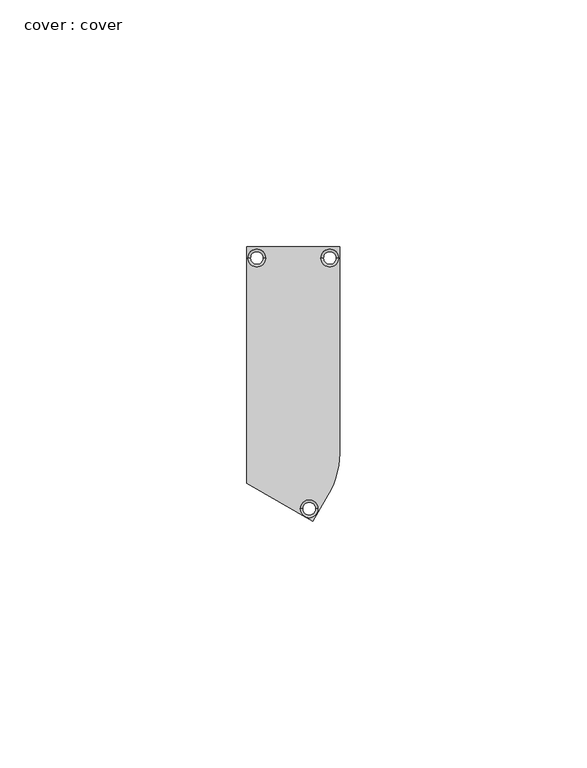
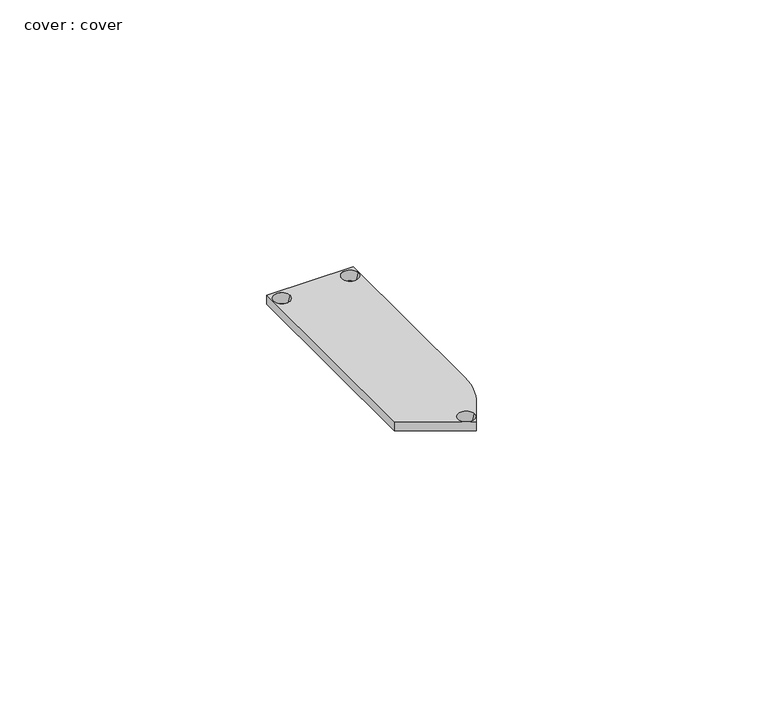
"""IFC4 building model written with IfcOpenShell, lengths in millimetres: proxy geometry, cover : cover."""

import ifcopenshell
import ifcopenshell.guid

model = None  # the IFC model being written
_history = None  # IfcOwnerHistory: only IFC2X3 demands one
_inside = {}  # id of a spatial element -> (the spatial element, [elements in it])
_under = {}  # id of a project, library or spatial element -> (it, [spatial elements below it])
_declared = {}  # id of a project -> (the project, [libraries it declares])
_typed = {}  # id of a type object -> (the type object, [elements of that type])
_made_of = {}  # id of a material, layer set ... -> (it, [elements and type objects made of it])


def new_model(schema):
    """Start an empty IFC model of exactly this schema.

    Asked for "IFC4X3", IfcOpenShell would pick the latest addendum, in which some entities
    have other attributes; the version numbers below select the first issue.
    IFC2X3 requires an IfcOwnerHistory on every rooted entity: one is made here for all.
    """
    global model, _history
    if schema == "IFC4X3":
        model = ifcopenshell.file(schema_version=(4, 3, 0, 0))
    else:
        model = ifcopenshell.file(schema=schema)
    _inside.clear()
    _under.clear()
    _declared.clear()
    _typed.clear()
    _made_of.clear()
    _history = None
    if model.schema == "IFC2X3":
        org = make("IfcOrganization", Name="unknown")
        user = make(
            "IfcPersonAndOrganization",
            ThePerson=make("IfcPerson", FamilyName="unknown"),
            TheOrganization=org,
        )
        app = make(
            "IfcApplication",
            ApplicationDeveloper=org,
            Version="unknown",
            ApplicationFullName="unknown",
            ApplicationIdentifier="unknown",
        )
        _history = make(
            "IfcOwnerHistory",
            OwningUser=user,
            OwningApplication=app,
            ChangeAction="ADDED",
            CreationDate=0,
        )
    return model


def make(cls, **values):
    """One entity of the class cls with the attributes given. An attribute that is None is left unset."""
    return model.create_entity(
        cls, **{name: value for name, value in values.items() if value is not None}
    )


def rooted(cls, **values):
    """An entity with a GlobalId (a new one), such as an element, a storey or a relation."""
    return make(cls, GlobalId=ifcopenshell.guid.new(), OwnerHistory=_history, **values)


def si_unit(unit_type, name, prefix=None):
    """IfcSIUnit, for example si_unit("LENGTHUNIT", "METRE", prefix="MILLI")."""
    return make("IfcSIUnit", UnitType=unit_type, Prefix=prefix, Name=name)


def assignment(units):
    """IfcUnitAssignment: the units of a project."""
    return None if units is None else make("IfcUnitAssignment", Units=units)


def point(xyz):
    """IfcCartesianPoint."""
    return None if xyz is None else make("IfcCartesianPoint", Coordinates=xyz)


def direction(xyz):
    """IfcDirection."""
    return None if xyz is None else make("IfcDirection", DirectionRatios=xyz)


def frame(location, z_axis=None, x_axis=None):
    """IfcAxis2Placement3D, a coordinate frame: its origin and axes. An axis left out is left unset."""
    return make(
        "IfcAxis2Placement3D",
        Location=point(location),
        Axis=direction(z_axis),
        RefDirection=direction(x_axis),
    )


def origin():
    """The frame at (0, 0, 0) with its axes left unset."""
    return frame((0.0, 0.0, 0.0))


def place(relative_to, where):
    """IfcLocalPlacement: puts the frame where relative to a parent placement (None: the world)."""
    return make(
        "IfcLocalPlacement", PlacementRelTo=relative_to, RelativePlacement=where
    )


def context(
    kind, dimensions, precision=None, world=None, true_north=None, identifier=None
):
    """IfcGeometricRepresentationContext, for example the 3D "Model" context."""
    return make(
        "IfcGeometricRepresentationContext",
        ContextIdentifier=identifier,
        ContextType=kind,
        CoordinateSpaceDimension=dimensions,
        Precision=precision,
        WorldCoordinateSystem=world,
        TrueNorth=true_north,
    )


def project(units=None, contexts=None):
    """IfcProject with its units and contexts."""
    return rooted(
        "IfcProject",
        Name="project",
        RepresentationContexts=contexts,
        UnitsInContext=assignment(units),
    )


def spatial(cls, under=None, at=None, **own):
    """A site, building, storey or space (cls), placed at a placement, below another one or the project."""
    s = rooted(cls, ObjectPlacement=at, **own)
    if under is not None:
        _under.setdefault(under.id(), (under, []))[1].append(s)
    return s


def polyline(points):
    """IfcPolyline through the points."""
    return make("IfcPolyline", Points=[point(p) for p in points])


def circle_curve(where, radius):
    """IfcCircle in the frame where."""
    return make("IfcCircle", Position=where, Radius=radius)


def shape(context_of_items, identifier, shape_type, items):
    """IfcShapeRepresentation: the items that make up one representation, for example the "Body"."""
    return make(
        "IfcShapeRepresentation",
        ContextOfItems=context_of_items,
        RepresentationIdentifier=identifier,
        RepresentationType=shape_type,
        Items=items,
    )


def source(mapping_origin, context_of_items, identifier, shape_type, items):
    """IfcRepresentationMap: a shape defined once, which mapped items show again and again."""
    return make(
        "IfcRepresentationMap",
        MappingOrigin=mapping_origin,
        MappedRepresentation=shape(context_of_items, identifier, shape_type, items),
    )


def transform(
    local_origin,
    x_axis=None,
    y_axis=None,
    z_axis=None,
    scale=None,
    scale2=None,
    scale3=None,
    uniform=True,
):
    """IfcCartesianTransformationOperator3D, or its non-uniform kind. x_axis, y_axis, z_axis: its Axis1, 2, 3."""
    if uniform:
        return make(
            "IfcCartesianTransformationOperator3D",
            Axis1=direction(x_axis),
            Axis2=direction(y_axis),
            LocalOrigin=point(local_origin),
            Scale=scale,
            Axis3=direction(z_axis),
        )
    return make(
        "IfcCartesianTransformationOperator3DnonUniform",
        Axis1=direction(x_axis),
        Axis2=direction(y_axis),
        LocalOrigin=point(local_origin),
        Scale=scale,
        Axis3=direction(z_axis),
        Scale2=scale2,
        Scale3=scale3,
    )


def mapped(mapping_source, mapping_target):
    """IfcMappedItem: shows the shape of a source again, moved by a transform."""
    return make(
        "IfcMappedItem", MappingSource=mapping_source, MappingTarget=mapping_target
    )


def made_of(thing, what):
    """Note that an element or type object is made of a material, layer set ...; save() writes the relation."""
    if what is not None:
        _made_of.setdefault(what.id(), (what, []))[1].append(thing)
    return thing


def element(
    cls,
    number,
    at=None,
    inside=None,
    cuts=None,
    type_object=None,
    material=None,
    context=None,
    identifier="Body",
    shape_type=None,
    held_by="IfcProductDefinitionShape",
    body=None,
    shapes=None,
    **own,
):
    """One element of the class cls, such as IfcWall. Its Tag is "e" and its number.

    at: its placement. inside: the storey or other place that contains it. cuts: it is an
    opening in that element (IfcRelVoidsElement). A single representation is given by context,
    identifier, shape_type and body (its items); several are given by shapes. held_by: the class
    of the entity that holds the representations. save() writes the other relations.
    """
    e = rooted(cls, Tag="e%d" % number, ObjectPlacement=at, **own)
    if body is not None:
        shapes = [shape(context, identifier, shape_type, body)]
    if shapes is not None:
        e.Representation = make(held_by, Representations=shapes)
    if inside is not None:
        _inside.setdefault(inside.id(), (inside, []))[1].append(e)
    if cuts is not None:
        rooted(
            "IfcRelVoidsElement", RelatingBuildingElement=cuts, RelatedOpeningElement=e
        )
    if type_object is not None:
        _typed.setdefault(type_object.id(), (type_object, []))[1].append(e)
    return made_of(e, material)


def aggregate(whole, parts):
    """IfcRelAggregates: a whole, such as a stair, and the parts it consists of."""
    return rooted("IfcRelAggregates", RelatingObject=whole, RelatedObjects=parts)


def save(model, path):
    """Write the relations noted so far, then the file.

    IfcRelAggregates (storeys below a building ...), IfcRelContainedInSpatialStructure (elements
    in a storey), IfcRelDefinesByType, IfcRelAssociatesMaterial and IfcRelDeclares: one each for
    every whole, place, type object, material and project.
    """
    for whole, parts in _under.values():
        aggregate(whole, parts)
    for where, things in _inside.values():
        rooted(
            "IfcRelContainedInSpatialStructure",
            RelatedElements=things,
            RelatingStructure=where,
        )
    for kind, things in _typed.values():
        rooted("IfcRelDefinesByType", RelatedObjects=things, RelatingType=kind)
    for what, things in _made_of.values():
        rooted("IfcRelAssociatesMaterial", RelatedObjects=things, RelatingMaterial=what)
    for by, libraries in _declared.values():
        rooted("IfcRelDeclares", RelatingContext=by, RelatedDefinitions=libraries)
    model.write(path)


def plane_surface(at):
    """IfcPlane: the flat surface through the origin of the frame at, square to its z axis."""
    return make("IfcPlane", Position=at)


def revolved_surface(curve, axis_point, axis_direction):
    """IfcSurfaceOfRevolution: the curve turned about the line through axis_point along axis_direction."""
    return make(
        "IfcSurfaceOfRevolution",
        SweptCurve=make("IfcArbitraryOpenProfileDef", ProfileType="CURVE", Curve=curve),
        AxisPosition=make("IfcAxis1Placement", Location=point(axis_point), Axis=direction(axis_direction)),
    )


def advanced_brep(points, edges, surfaces, faces):
    """IfcAdvancedBrep: a solid bounded by faces that lie on surfaces and meet in shared edges.

    An edge is (start, end): straight between two places in points (the first is 0);
    or (start, end, curve); or (start, end, curve, False) where it runs against its curve.
    A face is (place in surfaces, loops), or (place, loops, False) where it looks against
    its surface's normal. A loop lists edges by number (the first is 1), with a minus sign
    where the edge is run from its end to its start. The first loop is the outer one.
    """
    corners = [point(p) for p in points]
    vertices = [make("IfcVertexPoint", VertexGeometry=c) for c in corners]
    made = []
    for start, end, *more in edges:
        made.append(
            make(
                "IfcEdgeCurve",
                EdgeStart=vertices[start],
                EdgeEnd=vertices[end],
                EdgeGeometry=more[0] if more else make("IfcPolyline", Points=[corners[start], corners[end]]),
                SameSense=more[1] if len(more) > 1 else True,
            )
        )
    hull = []
    for where, loops, *sense in faces:
        bounds = []
        for j, loop in enumerate(loops):
            ring = [make("IfcOrientedEdge", EdgeElement=made[abs(k) - 1], Orientation=k > 0) for k in loop]
            bounds.append(
                make(
                    "IfcFaceOuterBound" if j == 0 else "IfcFaceBound",
                    Bound=make("IfcEdgeLoop", EdgeList=ring),
                    Orientation=True,
                )
            )
        hull.append(make("IfcAdvancedFace", Bounds=bounds, FaceSurface=surfaces[where], SameSense=sense[0] if sense else True))
    return make("IfcAdvancedBrep", Outer=make("IfcClosedShell", CfsFaces=hull))


def cover_cover_f3c25fb8(model_context):
    return source(origin(), model_context, "Body", "AdvancedBrep", [
        advanced_brep(
        [(4663.3311724, 3578.6670305, 2.0), (4663.3311724, 3530.8564939, 2.0), (4676.6686902, 3523.1530364, 2.0), (4680.3669524, 3529.5586705, 2.0), (4680.8851124, 3530.7118305, 2.0), (4681.3143724, 3531.9030905, 2.0), (4681.6547324, 3533.1222905, 2.0), (4681.9011124, 3534.3618105, 2.0), (4682.0560524, 3535.6191105, 2.0), (4682.1119324, 3536.8840305, 2.0), (4682.1119324, 3578.6670305, 2.0), (4667.1314224, 3576.4165905, 2.0), (4663.5314224, 3576.4165905, 2.0), (4681.9129524, 3576.4165905, 2.0), (4678.3129524, 3576.4165905, 2.0), (4677.7131366, 3525.6369105, 2.0), (4674.1587083, 3525.6369105, 2.0), (4663.3311724, 3578.6670305, 0.0), (4682.1119324, 3578.6670305, 0.0), (4682.1119324, 3536.8840305, 0.0), (4682.0560524, 3535.6191105, 0.0), (4681.9011124, 3534.3618105, 0.0), (4681.6547324, 3533.1222905, 0.0), (4681.3143724, 3531.9030905, 0.0), (4680.8851124, 3530.7118305, 0.0), (4680.3669524, 3529.5586705, 0.0), (4676.6686902, 3523.1530364, 0.0), (4663.3311724, 3530.8564939, 0.0), (4664.0314224, 3576.4165905, 0.0), (4666.6314224, 3576.4165905, 0.0), (4678.8129524, 3576.4165905, 0.0), (4681.4129524, 3576.4165905, 0.0), (4674.6206691, 3525.6369105, 0.0), (4677.2511758, 3525.6369105, 0.0)],
        [
            (0, 1),
            (1, 2),
            (2, 3),
            (3, 4),
            (4, 5),
            (5, 6),
            (6, 7),
            (7, 8),
            (8, 9),
            (9, 10),
            (10, 0),
            (11, 12, circle_curve(frame((4665.3314224, 3576.4165905, 2.0), z_axis=(0.0, 0.0, -1.0), x_axis=(-1.0, 0.0, 0.0)), 1.8)),
            (12, 11, circle_curve(frame((4665.3314224, 3576.4165905, 2.0), z_axis=(0.0, 0.0, -1.0), x_axis=(1.0, 0.0, 0.0)), 1.8)),
            (13, 14, circle_curve(frame((4680.1129524, 3576.4165905, 2.0), z_axis=(0.0, 0.0, -1.0), x_axis=(-1.0, 0.0, 0.0)), 1.8)),
            (14, 13, circle_curve(frame((4680.1129524, 3576.4165905, 2.0), z_axis=(0.0, 0.0, -1.0), x_axis=(1.0, 0.0, 0.0)), 1.8)),
            (15, 16, circle_curve(frame((4675.9359224, 3525.6369105, 2.0), z_axis=(0.0, 0.0, -1.0), x_axis=(-1.0, 0.0, 0.0)), 1.7772142)),
            (16, 15, circle_curve(frame((4675.9359224, 3525.6369105, 2.0), z_axis=(0.0, 0.0, -1.0), x_axis=(1.0, 0.0, 0.0)), 1.7772142)),
            (17, 18),
            (18, 19),
            (19, 20),
            (20, 21),
            (21, 22),
            (22, 23),
            (23, 24),
            (24, 25),
            (25, 26),
            (26, 27),
            (27, 17),
            (28, 29, circle_curve(frame((4665.3314224, 3576.4165905, 0.0), z_axis=(0.0, 0.0, 1.0), x_axis=(-1.0, 0.0, 0.0)), 1.3)),
            (29, 28, circle_curve(frame((4665.3314224, 3576.4165905, 0.0), z_axis=(0.0, 0.0, 1.0), x_axis=(1.0, 0.0, 0.0)), 1.3)),
            (30, 31, circle_curve(frame((4680.1129524, 3576.4165905, 0.0), z_axis=(0.0, 0.0, 1.0), x_axis=(-1.0, 0.0, 0.0)), 1.3)),
            (31, 30, circle_curve(frame((4680.1129524, 3576.4165905, 0.0), z_axis=(0.0, 0.0, 1.0), x_axis=(1.0, 0.0, 0.0)), 1.3)),
            (32, 33, circle_curve(frame((4675.9359224, 3525.6369105, 0.0), z_axis=(0.0, 0.0, 1.0), x_axis=(-1.0, 0.0, 0.0)), 1.3152534)),
            (33, 32, circle_curve(frame((4675.9359224, 3525.6369105, 0.0), z_axis=(0.0, 0.0, 1.0), x_axis=(1.0, 0.0, 0.0)), 1.3152534)),
            (0, 17),
            (27, 1),
            (26, 2),
            (25, 3),
            (9, 19),
            (18, 10),
            (24, 4),
            (23, 5),
            (22, 6),
            (21, 7),
            (20, 8),
            (28, 12),
            (11, 29),
            (30, 14),
            (13, 31),
            (32, 16),
            (15, 33),
        ],
        [
            plane_surface(frame((4663.3311724, 3531.8548305, 2.0), z_axis=(0.0, 0.0, 1.0), x_axis=(0.0, -1.0, 0.0))),
            plane_surface(frame((4663.3311724, 3531.8548305, 0.0), z_axis=(0.0, 0.0, -1.0), x_axis=(0.0, 1.0, 0.0))),
            plane_surface(frame((4663.3311724, 3578.6670305, 2.0), z_axis=(-1.0, 0.0, 0.0), x_axis=(0.0, 0.0, -1.0))),
            plane_surface(frame((4663.3311724, 3530.8564939, 2.0), z_axis=(-0.5001479267947538, -0.8659399813629751, 0.0), x_axis=(0.0, 0.0, -1.0))),
            plane_surface(frame((4676.6686902, 3523.1530364, 2.0), z_axis=(0.8660272939548952, -0.49999672611444335, 0.0), x_axis=(0.0, 0.0, -1.0))),
            plane_surface(frame((4682.1119324, 3536.8840305, 2.0), z_axis=(1.0, 0.0, 0.0), x_axis=(0.0, 0.0, -1.0))),
            plane_surface(frame((4680.3669524, 3529.5586705, 2.0), z_axis=(0.91214692510674, -0.40986337603928397, 0.0), x_axis=(0.0, 0.0, -1.0))),
            plane_surface(frame((4680.8851124, 3530.7118305, 2.0), z_axis=(0.9407850831608502, -0.3390035800725891, 0.0), x_axis=(0.0, 0.0, -1.0))),
            plane_surface(frame((4681.3143724, 3531.9030905, 2.0), z_axis=(0.9631721335643817, -0.26888555395379093, 0.0), x_axis=(0.0, 0.0, -1.0))),
            plane_surface(frame((4681.6547324, 3533.1222905, 2.0), z_axis=(0.9808118970912181, -0.19495646315094542, 0.0), x_axis=(0.0, 0.0, -1.0))),
            plane_surface(frame((4681.9011124, 3534.3618105, 2.0), z_axis=(0.9924922999614717, -0.12230713191465294, 0.0), x_axis=(0.0, 0.0, -1.0))),
            plane_surface(frame((4682.0560524, 3535.6191105, 2.0), z_axis=(0.9990256352193916, -0.04413366260000536, 0.0), x_axis=(0.0, 0.0, -1.0))),
            plane_surface(frame((4682.1119324, 3578.6670305, 2.0), z_axis=(0.0, 1.0, 0.0), x_axis=(0.0, 0.0, -1.0))),
            revolved_surface(polyline([(4663.5314224, 3576.4165905, 2.0), (4664.0314224, 3576.4165905, 0.0)]), (4665.3314224, 3576.4165905, -5.2), (0.0, 0.0, 1.0)),
            revolved_surface(polyline([(4678.3129524, 3576.4165905, 2.0), (4678.8129524, 3576.4165905, 0.0)]), (4680.1129524, 3576.4165905, -5.2), (0.0, 0.0, 1.0)),
            revolved_surface(polyline([(4674.1587083, 3525.6369105, 2.0), (4674.620669086516, 3525.6369105, 0.0)]), (4675.9359224, 3525.6369105, -5.6942206), (0.0, 0.0, 1.0)),
        ],
        [
            (0, [[1, 2, 3, 4, 5, 6, 7, 8, 9, 10, 11], [12, 13], [14, 15], [16, 17]]),
            (1, [[18, 19, 20, 21, 22, 23, 24, 25, 26, 27, 28], [29, 30], [31, 32], [33, 34]]),
            (2, [[-1, 35, -28, 36]]),
            (3, [[-2, -36, -27, 37]]),
            (4, [[-3, -37, -26, 38]]),
            (5, [[-10, 39, -19, 40]]),
            (6, [[-4, -38, -25, 41]]),
            (7, [[-5, -41, -24, 42]]),
            (8, [[-6, -42, -23, 43]]),
            (9, [[-7, -43, -22, 44]]),
            (10, [[-8, -44, -21, 45]]),
            (11, [[-9, -45, -20, -39]]),
            (12, [[-11, -40, -18, -35]]),
            (13, [[46, -12, 47, -29]]),
            (13, [[-46, -30, -47, -13]]),
            (14, [[48, -14, 49, -31]]),
            (14, [[-48, -32, -49, -15]]),
            (15, [[50, -16, 51, -33]]),
            (15, [[-50, -34, -51, -17]]),
        ],
    ),
    ])


if __name__ == "__main__":
    model = new_model("IFC4")
    model_context = context("Model", 3, world=origin())
    ifc_project = project(units=[si_unit("LENGTHUNIT", "METRE", prefix="MILLI")], contexts=[model_context])
    site = spatial("IfcSite", under=ifc_project)
    building = spatial("IfcBuilding", under=site)
    placement = place(None, origin())
    cover_cover_shape = cover_cover_f3c25fb8(model_context)
    element("IfcBuildingElementProxy", 1, Name="cover : cover", ObjectType="cover : cover", at=placement, inside=building, context=model_context, shape_type="MappedRepresentation", body=[
        mapped(cover_cover_shape, transform((0.0, 0.0, 0.0), x_axis=(1.0, 0.0, 0.0), y_axis=(0.0, 1.0, 0.0), z_axis=(0.0, 0.0, 1.0))),
    ])
    save(model, "model.ifc")

# Revit data of these elements
# Project information
#   Data de emissão do projeto = "Data de emissão"
#   Status do projeto = "Status do projeto"
#   Nome do cliente = "Proprietário"
#   Endereço do projeto = "Insira aqui o endereço"
#   Nome do projeto = "Nome do projeto"
#   Número do projeto = "0001"
